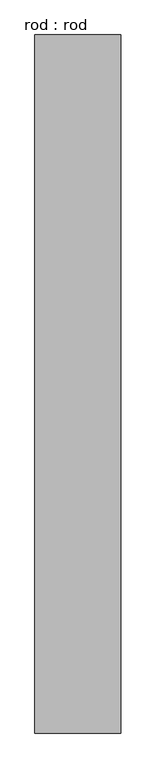
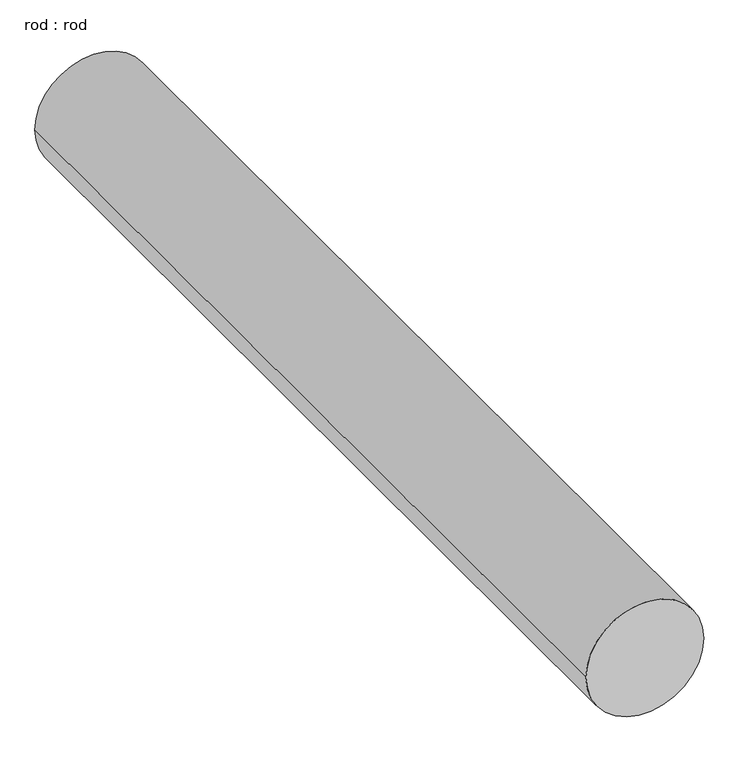
"""IFC4 building model written with IfcOpenShell, lengths in millimetres: proxy geometry, rod : rod."""

import ifcopenshell
import ifcopenshell.guid

model = None  # the IFC model being written
_history = None  # IfcOwnerHistory: only IFC2X3 demands one
_inside = {}  # id of a spatial element -> (the spatial element, [elements in it])
_under = {}  # id of a project, library or spatial element -> (it, [spatial elements below it])
_declared = {}  # id of a project -> (the project, [libraries it declares])
_typed = {}  # id of a type object -> (the type object, [elements of that type])
_made_of = {}  # id of a material, layer set ... -> (it, [elements and type objects made of it])


def new_model(schema):
    """Start an empty IFC model of exactly this schema.

    Asked for "IFC4X3", IfcOpenShell would pick the latest addendum, in which some entities
    have other attributes; the version numbers below select the first issue.
    IFC2X3 requires an IfcOwnerHistory on every rooted entity: one is made here for all.
    """
    global model, _history
    if schema == "IFC4X3":
        model = ifcopenshell.file(schema_version=(4, 3, 0, 0))
    else:
        model = ifcopenshell.file(schema=schema)
    _inside.clear()
    _under.clear()
    _declared.clear()
    _typed.clear()
    _made_of.clear()
    _history = None
    if model.schema == "IFC2X3":
        org = make("IfcOrganization", Name="unknown")
        user = make(
            "IfcPersonAndOrganization",
            ThePerson=make("IfcPerson", FamilyName="unknown"),
            TheOrganization=org,
        )
        app = make(
            "IfcApplication",
            ApplicationDeveloper=org,
            Version="unknown",
            ApplicationFullName="unknown",
            ApplicationIdentifier="unknown",
        )
        _history = make(
            "IfcOwnerHistory",
            OwningUser=user,
            OwningApplication=app,
            ChangeAction="ADDED",
            CreationDate=0,
        )
    return model


def make(cls, **values):
    """One entity of the class cls with the attributes given. An attribute that is None is left unset."""
    return model.create_entity(
        cls, **{name: value for name, value in values.items() if value is not None}
    )


def rooted(cls, **values):
    """An entity with a GlobalId (a new one), such as an element, a storey or a relation."""
    return make(cls, GlobalId=ifcopenshell.guid.new(), OwnerHistory=_history, **values)


def si_unit(unit_type, name, prefix=None):
    """IfcSIUnit, for example si_unit("LENGTHUNIT", "METRE", prefix="MILLI")."""
    return make("IfcSIUnit", UnitType=unit_type, Prefix=prefix, Name=name)


def assignment(units):
    """IfcUnitAssignment: the units of a project."""
    return None if units is None else make("IfcUnitAssignment", Units=units)


def point(xyz):
    """IfcCartesianPoint."""
    return None if xyz is None else make("IfcCartesianPoint", Coordinates=xyz)


def direction(xyz):
    """IfcDirection."""
    return None if xyz is None else make("IfcDirection", DirectionRatios=xyz)


def frame(location, z_axis=None, x_axis=None):
    """IfcAxis2Placement3D, a coordinate frame: its origin and axes. An axis left out is left unset."""
    return make(
        "IfcAxis2Placement3D",
        Location=point(location),
        Axis=direction(z_axis),
        RefDirection=direction(x_axis),
    )


def frame_2d(location, x_axis=None):
    """IfcAxis2Placement2D, a coordinate frame in the plane: its origin and x axis."""
    return make(
        "IfcAxis2Placement2D", Location=point(location), RefDirection=direction(x_axis)
    )


def origin():
    """The frame at (0, 0, 0) with its axes left unset."""
    return frame((0.0, 0.0, 0.0))


def place(relative_to, where):
    """IfcLocalPlacement: puts the frame where relative to a parent placement (None: the world)."""
    return make(
        "IfcLocalPlacement", PlacementRelTo=relative_to, RelativePlacement=where
    )


def context(
    kind, dimensions, precision=None, world=None, true_north=None, identifier=None
):
    """IfcGeometricRepresentationContext, for example the 3D "Model" context."""
    return make(
        "IfcGeometricRepresentationContext",
        ContextIdentifier=identifier,
        ContextType=kind,
        CoordinateSpaceDimension=dimensions,
        Precision=precision,
        WorldCoordinateSystem=world,
        TrueNorth=true_north,
    )


def project(units=None, contexts=None):
    """IfcProject with its units and contexts."""
    return rooted(
        "IfcProject",
        Name="project",
        RepresentationContexts=contexts,
        UnitsInContext=assignment(units),
    )


def spatial(cls, under=None, at=None, **own):
    """A site, building, storey or space (cls), placed at a placement, below another one or the project."""
    s = rooted(cls, ObjectPlacement=at, **own)
    if under is not None:
        _under.setdefault(under.id(), (under, []))[1].append(s)
    return s


def circle_curve(where, radius):
    """IfcCircle in the frame where."""
    return make("IfcCircle", Position=where, Radius=radius)


def trimmed(basis, trim1, trim2, sense, master):
    """IfcTrimmedCurve: the piece of a basis curve between two trims."""
    return make(
        "IfcTrimmedCurve",
        BasisCurve=basis,
        Trim1=trim1,
        Trim2=trim2,
        SenseAgreement=sense,
        MasterRepresentation=master,
    )


def segment(curve, same_sense, transition):
    """IfcCompositeCurveSegment."""
    return make(
        "IfcCompositeCurveSegment",
        Transition=transition,
        SameSense=same_sense,
        ParentCurve=curve,
    )


def composite_curve(segments, self_intersect=None):
    """IfcCompositeCurve: segments joined end to end."""
    return make("IfcCompositeCurve", Segments=segments, SelfIntersect=self_intersect)


def outline(outer, holes=None, kind="AREA"):
    """IfcArbitraryClosedProfileDef: a profile drawn as a closed curve; with holes, ...WithVoids."""
    if holes is None:
        return make("IfcArbitraryClosedProfileDef", ProfileType=kind, OuterCurve=outer)
    return make(
        "IfcArbitraryProfileDefWithVoids",
        ProfileType=kind,
        OuterCurve=outer,
        InnerCurves=holes,
    )


def extrude(swept, where, along, depth):
    """IfcExtrudedAreaSolid: the profile swept, set in the frame where, extruded along a direction by depth."""
    return make(
        "IfcExtrudedAreaSolid",
        SweptArea=swept,
        Position=where,
        ExtrudedDirection=direction(along),
        Depth=depth,
    )


def shape(context_of_items, identifier, shape_type, items):
    """IfcShapeRepresentation: the items that make up one representation, for example the "Body"."""
    return make(
        "IfcShapeRepresentation",
        ContextOfItems=context_of_items,
        RepresentationIdentifier=identifier,
        RepresentationType=shape_type,
        Items=items,
    )


def source(mapping_origin, context_of_items, identifier, shape_type, items):
    """IfcRepresentationMap: a shape defined once, which mapped items show again and again."""
    return make(
        "IfcRepresentationMap",
        MappingOrigin=mapping_origin,
        MappedRepresentation=shape(context_of_items, identifier, shape_type, items),
    )


def transform(
    local_origin,
    x_axis=None,
    y_axis=None,
    z_axis=None,
    scale=None,
    scale2=None,
    scale3=None,
    uniform=True,
):
    """IfcCartesianTransformationOperator3D, or its non-uniform kind. x_axis, y_axis, z_axis: its Axis1, 2, 3."""
    if uniform:
        return make(
            "IfcCartesianTransformationOperator3D",
            Axis1=direction(x_axis),
            Axis2=direction(y_axis),
            LocalOrigin=point(local_origin),
            Scale=scale,
            Axis3=direction(z_axis),
        )
    return make(
        "IfcCartesianTransformationOperator3DnonUniform",
        Axis1=direction(x_axis),
        Axis2=direction(y_axis),
        LocalOrigin=point(local_origin),
        Scale=scale,
        Axis3=direction(z_axis),
        Scale2=scale2,
        Scale3=scale3,
    )


def mapped(mapping_source, mapping_target):
    """IfcMappedItem: shows the shape of a source again, moved by a transform."""
    return make(
        "IfcMappedItem", MappingSource=mapping_source, MappingTarget=mapping_target
    )


def made_of(thing, what):
    """Note that an element or type object is made of a material, layer set ...; save() writes the relation."""
    if what is not None:
        _made_of.setdefault(what.id(), (what, []))[1].append(thing)
    return thing


def element(
    cls,
    number,
    at=None,
    inside=None,
    cuts=None,
    type_object=None,
    material=None,
    context=None,
    identifier="Body",
    shape_type=None,
    held_by="IfcProductDefinitionShape",
    body=None,
    shapes=None,
    **own,
):
    """One element of the class cls, such as IfcWall. Its Tag is "e" and its number.

    at: its placement. inside: the storey or other place that contains it. cuts: it is an
    opening in that element (IfcRelVoidsElement). A single representation is given by context,
    identifier, shape_type and body (its items); several are given by shapes. held_by: the class
    of the entity that holds the representations. save() writes the other relations.
    """
    e = rooted(cls, Tag="e%d" % number, ObjectPlacement=at, **own)
    if body is not None:
        shapes = [shape(context, identifier, shape_type, body)]
    if shapes is not None:
        e.Representation = make(held_by, Representations=shapes)
    if inside is not None:
        _inside.setdefault(inside.id(), (inside, []))[1].append(e)
    if cuts is not None:
        rooted(
            "IfcRelVoidsElement", RelatingBuildingElement=cuts, RelatedOpeningElement=e
        )
    if type_object is not None:
        _typed.setdefault(type_object.id(), (type_object, []))[1].append(e)
    return made_of(e, material)


def aggregate(whole, parts):
    """IfcRelAggregates: a whole, such as a stair, and the parts it consists of."""
    return rooted("IfcRelAggregates", RelatingObject=whole, RelatedObjects=parts)


def save(model, path):
    """Write the relations noted so far, then the file.

    IfcRelAggregates (storeys below a building ...), IfcRelContainedInSpatialStructure (elements
    in a storey), IfcRelDefinesByType, IfcRelAssociatesMaterial and IfcRelDeclares: one each for
    every whole, place, type object, material and project.
    """
    for whole, parts in _under.values():
        aggregate(whole, parts)
    for where, things in _inside.values():
        rooted(
            "IfcRelContainedInSpatialStructure",
            RelatedElements=things,
            RelatingStructure=where,
        )
    for kind, things in _typed.values():
        rooted("IfcRelDefinesByType", RelatedObjects=things, RelatingType=kind)
    for what, things in _made_of.values():
        rooted("IfcRelAssociatesMaterial", RelatedObjects=things, RelatingMaterial=what)
    for by, libraries in _declared.values():
        rooted("IfcRelDeclares", RelatingContext=by, RelatedDefinitions=libraries)
    model.write(path)


def rod_rod_ca3cc784(model_context):
    return source(origin(), model_context, "Body", "SweptSolid", [
        extrude(outline(composite_curve([segment(trimmed(circle_curve(frame_2d((0.0108462, 0.0)), 200.0), [point((0.0108462, 200.0))], [point((0.0108462, -200.0))], False, "CARTESIAN"), True, "CONTINUOUS"), segment(trimmed(circle_curve(frame_2d((0.0108462, 0.0)), 200.0), [point((0.0108462, -200.0))], [point((0.0108462, 200.0))], False, "CARTESIAN"), True, "CONTINUOUS")], self_intersect=False)), frame((0.0, 2469.5143296, 0.0), z_axis=(0.0, 1.0, 0.0), x_axis=(0.0, 0.0, 1.0)), (0.0, 0.0, 1.0), 3246.4285714),
    ])


if __name__ == "__main__":
    model = new_model("IFC4")
    model_context = context("Model", 3, world=origin())
    ifc_project = project(units=[si_unit("LENGTHUNIT", "METRE", prefix="MILLI")], contexts=[model_context])
    site = spatial("IfcSite", under=ifc_project)
    building = spatial("IfcBuilding", under=site)
    placement = place(None, origin())
    rod_rod_shape = rod_rod_ca3cc784(model_context)
    element("IfcBuildingElementProxy", 1, Name="rod : rod", ObjectType="rod : rod", at=placement, inside=building, context=model_context, shape_type="MappedRepresentation", body=[
        mapped(rod_rod_shape, transform((0.0, 0.0, 0.0), x_axis=(1.0, 0.0, 0.0), y_axis=(0.0, 1.0, 0.0), z_axis=(0.0, 0.0, 1.0))),
    ])
    save(model, "model.ifc")

# Revit data of these elements
# Type "rod : rod"
#   Default Elevation = 0
